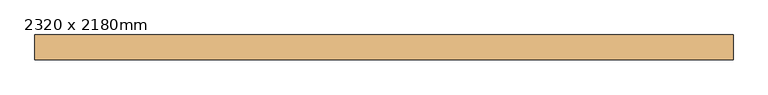
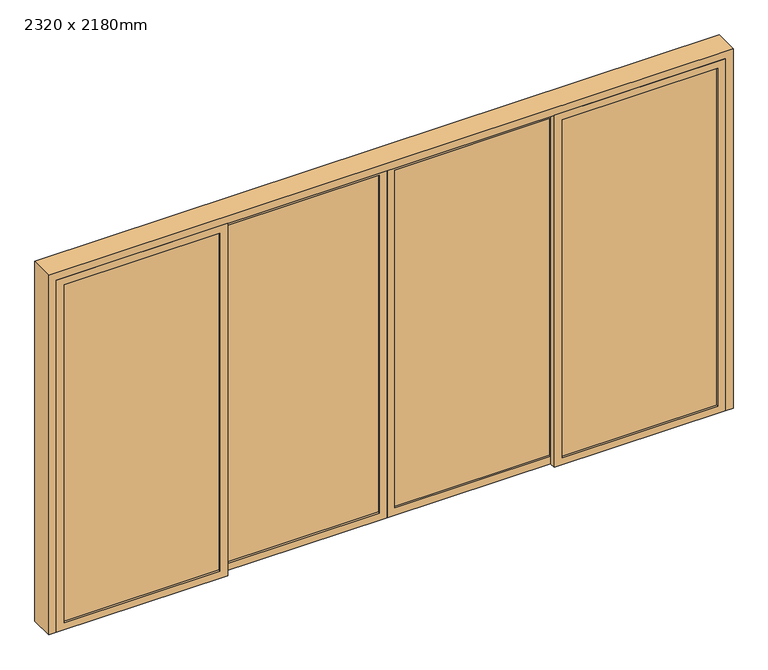
"""IFC4 building model written with IfcOpenShell, lengths in millimetres: door geometry, Porta envidraçada de correr quádrupla sem revestimento : 2320 x 2180mm."""

from ifc_helpers import new_model, si_unit, point, frame, frame_2d, origin, place, context, project, spatial, polyline, circle_curve, trimmed, segment, composite_curve, outline, extrude, source, transform, mapped, element, save


def door_2320_x_2180mm_da102013(model_context):
    return source(origin(), model_context, "Body", "SweptSolid", [
        extrude(outline(composite_curve([segment(trimmed(circle_curve(frame_2d((990.0, 15.0)), 10.0), [point((1000.0, 15.0))], [point((990.0, 5.0))], False, "CARTESIAN"), True, "CONTINUOUS"), segment(polyline([(990.0, 5.0), (810.0, 5.0)]), True, "CONTINUOUS"), segment(trimmed(circle_curve(frame_2d((810.0, 15.0)), 10.0), [point((810.0, 5.0))], [point((800.0, 15.0))], False, "CARTESIAN"), True, "CONTINUOUS"), segment(polyline([(800.0, 15.0), (800.0, 35.0)]), True, "CONTINUOUS"), segment(trimmed(circle_curve(frame_2d((810.0, 35.0)), 10.0), [point((800.0, 35.0))], [point((810.0, 45.0))], False, "CARTESIAN"), True, "CONTINUOUS"), segment(polyline([(810.0, 45.0), (990.0, 45.0)]), True, "CONTINUOUS"), segment(trimmed(circle_curve(frame_2d((990.0, 35.0)), 10.0), [point((990.0, 45.0))], [point((1000.0, 35.0))], False, "CARTESIAN"), True, "CONTINUOUS"), segment(polyline([(1000.0, 35.0), (1000.0, 15.0)]), True, "CONTINUOUS")], self_intersect=False), holes=[composite_curve([segment(trimmed(circle_curve(frame_2d((985.0, 25.0)), 5.0), [point((985.0, 20.0))], [point((985.0, 30.0))], True, "CARTESIAN"), True, "CONTINUOUS"), segment(trimmed(circle_curve(frame_2d((985.0, 25.0)), 5.0), [point((985.0, 30.0))], [point((985.0, 20.0))], True, "CARTESIAN"), True, "CONTINUOUS")], self_intersect=False), composite_curve([segment(trimmed(circle_curve(frame_2d((815.0, 25.0)), 5.0), [point((815.0, 20.0))], [point((815.0, 30.0))], True, "CARTESIAN"), True, "CONTINUOUS"), segment(trimmed(circle_curve(frame_2d((815.0, 25.0)), 5.0), [point((815.0, 30.0))], [point((815.0, 20.0))], True, "CARTESIAN"), True, "CONTINUOUS")], self_intersect=False), composite_curve([segment(polyline([(960.0, 15.0), (960.0, 35.0)]), True, "CONTINUOUS"), segment(trimmed(circle_curve(frame_2d((955.0, 35.0)), 5.0), [point((960.0, 35.0))], [point((955.0, 40.0))], True, "CARTESIAN"), True, "CONTINUOUS"), segment(polyline([(955.0, 40.0), (845.0, 40.0)]), True, "CONTINUOUS"), segment(trimmed(circle_curve(frame_2d((845.0, 35.0)), 5.0), [point((845.0, 40.0))], [point((840.0, 35.0))], True, "CARTESIAN"), True, "CONTINUOUS"), segment(polyline([(840.0, 35.0), (840.0, 15.0)]), True, "CONTINUOUS"), segment(trimmed(circle_curve(frame_2d((845.0, 15.0)), 5.0), [point((840.0, 15.0))], [point((845.0, 10.0))], True, "CARTESIAN"), True, "CONTINUOUS"), segment(polyline([(845.0, 10.0), (955.0, 10.0)]), True, "CONTINUOUS"), segment(trimmed(circle_curve(frame_2d((955.0, 15.0)), 5.0), [point((955.0, 10.0))], [point((960.0, 15.0))], True, "CARTESIAN"), True, "CONTINUOUS")], self_intersect=False)]), frame((0.0, 5.4, 0.0), z_axis=(0.0, 1.0, 0.0), x_axis=(0.0, 0.0, 1.0)), (0.0, 0.0, 1.0), 3.0),
        extrude(outline(composite_curve([segment(trimmed(circle_curve(frame_2d((990.0, -35.0)), 10.0), [point((1000.0, -35.0))], [point((990.0, -45.0))], False, "CARTESIAN"), True, "CONTINUOUS"), segment(polyline([(990.0, -45.0), (810.0, -45.0)]), True, "CONTINUOUS"), segment(trimmed(circle_curve(frame_2d((810.0, -35.0)), 10.0), [point((810.0, -45.0))], [point((800.0, -35.0))], False, "CARTESIAN"), True, "CONTINUOUS"), segment(polyline([(800.0, -35.0), (800.0, -15.0)]), True, "CONTINUOUS"), segment(trimmed(circle_curve(frame_2d((810.0, -15.0)), 10.0), [point((800.0, -15.0))], [point((810.0, -5.0))], False, "CARTESIAN"), True, "CONTINUOUS"), segment(polyline([(810.0, -5.0), (990.0, -5.0)]), True, "CONTINUOUS"), segment(trimmed(circle_curve(frame_2d((990.0, -15.0)), 10.0), [point((990.0, -5.0))], [point((1000.0, -15.0))], False, "CARTESIAN"), True, "CONTINUOUS"), segment(polyline([(1000.0, -15.0), (1000.0, -35.0)]), True, "CONTINUOUS")], self_intersect=False), holes=[composite_curve([segment(trimmed(circle_curve(frame_2d((985.0, -25.0)), 5.0), [point((985.0, -30.0))], [point((985.0, -20.0))], True, "CARTESIAN"), True, "CONTINUOUS"), segment(trimmed(circle_curve(frame_2d((985.0, -25.0)), 5.0), [point((985.0, -20.0))], [point((985.0, -30.0))], True, "CARTESIAN"), True, "CONTINUOUS")], self_intersect=False), composite_curve([segment(trimmed(circle_curve(frame_2d((815.0, -25.0)), 5.0), [point((815.0, -30.0))], [point((815.0, -20.0))], True, "CARTESIAN"), True, "CONTINUOUS"), segment(trimmed(circle_curve(frame_2d((815.0, -25.0)), 5.0), [point((815.0, -20.0))], [point((815.0, -30.0))], True, "CARTESIAN"), True, "CONTINUOUS")], self_intersect=False), composite_curve([segment(polyline([(960.0, -35.0), (960.0, -15.0)]), True, "CONTINUOUS"), segment(trimmed(circle_curve(frame_2d((955.0, -15.0)), 5.0), [point((960.0, -15.0))], [point((955.0, -10.0))], True, "CARTESIAN"), True, "CONTINUOUS"), segment(polyline([(955.0, -10.0), (845.0, -10.0)]), True, "CONTINUOUS"), segment(trimmed(circle_curve(frame_2d((845.0, -15.0)), 5.0), [point((845.0, -10.0))], [point((840.0, -15.0))], True, "CARTESIAN"), True, "CONTINUOUS"), segment(polyline([(840.0, -15.0), (840.0, -35.0)]), True, "CONTINUOUS"), segment(trimmed(circle_curve(frame_2d((845.0, -35.0)), 5.0), [point((840.0, -35.0))], [point((845.0, -40.0))], True, "CARTESIAN"), True, "CONTINUOUS"), segment(polyline([(845.0, -40.0), (955.0, -40.0)]), True, "CONTINUOUS"), segment(trimmed(circle_curve(frame_2d((955.0, -35.0)), 5.0), [point((955.0, -40.0))], [point((960.0, -35.0))], True, "CARTESIAN"), True, "CONTINUOUS")], self_intersect=False)]), frame((0.0, 5.4, 0.0), z_axis=(0.0, 1.0, 0.0), x_axis=(0.0, 0.0, 1.0)), (0.0, 0.0, 1.0), 3.0),
        extrude(outline(polyline([(2450.0, -1125.0), (0.0, -1125.0), (0.0, 0.0), (2450.0, 0.0), (2450.0, -1125.0)]), holes=[polyline([(2400.0, -50.0), (50.0, -50.0), (50.0, -1075.0), (2400.0, -1075.0), (2400.0, -50.0)])]), frame((0.0, -34.6, 0.0), z_axis=(0.0, 1.0, 0.0), x_axis=(0.0, 0.0, 1.0)), (0.0, 0.0, 1.0), 40.0),
        extrude(outline(polyline([(2450.0, 1075.0), (0.0, 1075.0), (0.0, 2200.0), (2450.0, 2200.0), (2450.0, 1075.0)]), holes=[polyline([(2400.0, 2150.0), (50.0, 2150.0), (50.0, 1125.0), (2400.0, 1125.0), (2400.0, 2150.0)])]), frame((0.0, -79.6, 0.0), z_axis=(0.0, 1.0, 0.0), x_axis=(0.0, 0.0, 1.0)), (0.0, 0.0, 1.0), 40.0),
        extrude(outline(polyline([(2450.0, 0.0), (0.0, 0.0), (0.0, 1125.0), (2450.0, 1125.0), (2450.0, 0.0)]), holes=[polyline([(2400.0, 1075.0), (50.0, 1075.0), (50.0, 50.0), (2400.0, 50.0), (2400.0, 1075.0)])]), frame((0.0, -34.6, 0.0), z_axis=(0.0, 1.0, 0.0), x_axis=(0.0, 0.0, 1.0)), (0.0, 0.0, 1.0), 40.0),
        extrude(outline(polyline([(2450.0, -2200.0), (0.0, -2200.0), (0.0, -1075.0), (2450.0, -1075.0), (2450.0, -2200.0)]), holes=[polyline([(2400.0, -1125.0), (50.0, -1125.0), (50.0, -2150.0), (2400.0, -2150.0), (2400.0, -1125.0)])]), frame((0.0, -79.6, 0.0), z_axis=(0.0, 1.0, 0.0), x_axis=(0.0, 0.0, 1.0)), (0.0, 0.0, 1.0), 40.0),
        extrude(outline(polyline([(0.0, 2200.0), (0.0, 2250.0), (2500.0, 2250.0), (2500.0, -2250.0), (0.0, -2250.0), (0.0, -2200.0), (2450.0, -2200.0), (2450.0, 2200.0), (0.0, 2200.0)])), frame((0.0, -79.6, 0.0), z_axis=(0.0, 1.0, 0.0), x_axis=(0.0, 0.0, 1.0)), (0.0, 0.0, 1.0), 159.2),
        extrude(outline(polyline([(1075.0, -7.6), (1075.0, -21.6), (50.0, -21.6), (50.0, -7.6), (1075.0, -7.6)])), frame((0.0, 0.0, 50.0), z_axis=(0.0, 0.0, 1.0), x_axis=(1.0, 0.0, 0.0)), (0.0, 0.0, 1.0), 2350.0),
        extrude(outline(polyline([(2150.0, -52.6), (2150.0, -66.6), (1125.0, -66.6), (1125.0, -52.6), (2150.0, -52.6)])), frame((0.0, 0.0, 50.0), z_axis=(0.0, 0.0, 1.0), x_axis=(1.0, 0.0, 0.0)), (0.0, 0.0, 1.0), 2350.0),
        extrude(outline(polyline([(-1125.0, -52.6), (-1125.0, -66.6), (-2150.0, -66.6), (-2150.0, -52.6), (-1125.0, -52.6)])), frame((0.0, 0.0, 50.0), z_axis=(0.0, 0.0, 1.0), x_axis=(1.0, 0.0, 0.0)), (0.0, 0.0, 1.0), 2350.0),
        extrude(outline(polyline([(-50.0, -7.6), (-50.0, -21.6), (-1075.0, -21.6), (-1075.0, -7.6), (-50.0, -7.6)])), frame((0.0, 0.0, 50.0), z_axis=(0.0, 0.0, 1.0), x_axis=(1.0, 0.0, 0.0)), (0.0, 0.0, 1.0), 2350.0),
        extrude(outline(polyline([(-1125.0, -52.6), (-1125.0, -66.6), (-2150.0, -66.6), (-2150.0, -52.6), (-1125.0, -52.6)])), frame((0.0, 0.0, 50.0), z_axis=(0.0, 0.0, 1.0), x_axis=(1.0, 0.0, 0.0)), (0.0, 0.0, 1.0), 2350.0),
        extrude(outline(polyline([(-50.0, -7.6), (-50.0, -21.6), (-1075.0, -21.6), (-1075.0, -7.6), (-50.0, -7.6)])), frame((0.0, 0.0, 50.0), z_axis=(0.0, 0.0, 1.0), x_axis=(1.0, 0.0, 0.0)), (0.0, 0.0, 1.0), 2350.0),
        extrude(outline(polyline([(1125.0, -52.6), (2150.0, -52.6), (2150.0, -66.6), (1125.0, -66.6), (1125.0, -52.6)])), frame((0.0, 0.0, 50.0), z_axis=(0.0, 0.0, 1.0), x_axis=(1.0, 0.0, 0.0)), (0.0, 0.0, 1.0), 2350.0),
        extrude(outline(polyline([(50.0, -7.6), (1075.0, -7.6), (1075.0, -21.6), (50.0, -21.6), (50.0, -7.6)])), frame((0.0, 0.0, 50.0), z_axis=(0.0, 0.0, 1.0), x_axis=(1.0, 0.0, 0.0)), (0.0, 0.0, 1.0), 2350.0),
    ])


if __name__ == "__main__":
    model = new_model("IFC4")
    model_context = context("Model", 3, world=origin())
    ifc_project = project(units=[si_unit("LENGTHUNIT", "METRE", prefix="MILLI")], contexts=[model_context])
    site = spatial("IfcSite", under=ifc_project)
    building = spatial("IfcBuilding", under=site)
    placement = place(None, origin())
    door_2320_x_2180mm_shape = door_2320_x_2180mm_da102013(model_context)
    element("IfcDoor", 1, ObjectType="Porta envidraçada de correr quádrupla sem revestimento : 2320 x 2180mm", at=placement, inside=building, context=model_context, shape_type="MappedRepresentation", body=[
        mapped(door_2320_x_2180mm_shape, transform((0.0, 0.0, 0.0), x_axis=(1.0, 0.0, 0.0), y_axis=(0.0, 1.0, 0.0), z_axis=(0.0, 0.0, 1.0))),
    ])
    save(model, "model.ifc")

# Revit data of these elements
# Type "Porta envidraçada de correr quádrupla sem revestimento : 2320 x 2180mm"
#   Type Mark = "P50"
#   Construction Type Id = "GSP4R"
#   Analytic Construction = "Vidraça única Pilkington 1/8 pol"
#   Visual Light Transmittance = 0.9
#   Solar Heat Gain Coefficient = 0.78
#   Rough Width = 4.50 m
#   Rough Height = 2.50 m
#   Largura da moldura do painel = 0.05 m
#   Espessura da moldura do painel = 0.04 m
#   Heat Transfer Coefficient (U) = 3.6886 W/(m²·K)
#   Largura da maçaneta = 0.04 m
#   Altura do puxador = 0.20 m
#   Largura da estrutura = 0.05 m
#   Height = 2.50 m
#   Width = 4.50 m
#   Function = 1
#   Material do puxador = none
#   Vidro = Vidro - Janela
#   Material da estrutura = Aluminum Sill
#   Thickness = 0
#   Wall Closure = (empty or 0)
# Element 1 (IfcDoor, "Porta envidraçada de correr quádrupla sem revestimento : 2320 x 2180mm")
#   Materials on its faces: "Aluminum Sill", "Vidro - Janela"
# Materials
#   "Vidro - Janela": class "Vidro", colour RGB 249 249 249, transparency 1, Cost = 0
#   "Aluminum Sill": class "Não atribuído", colour RGB 247 247 247, transparency 0
